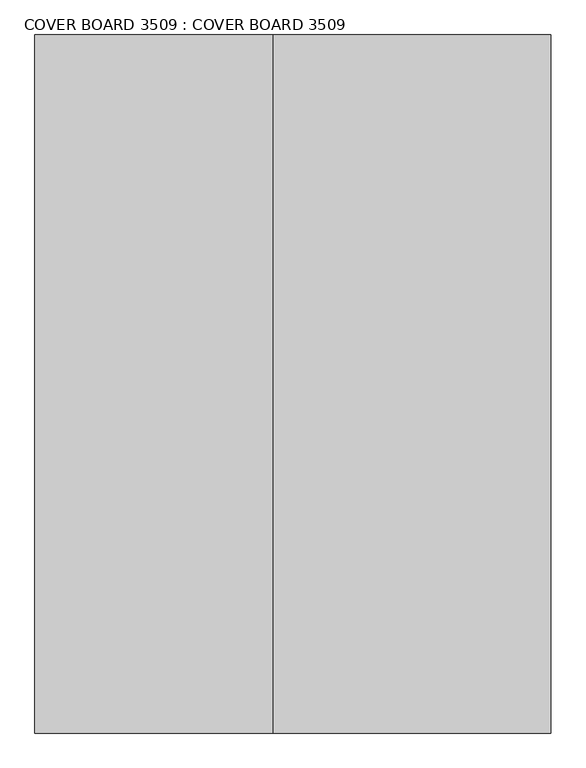
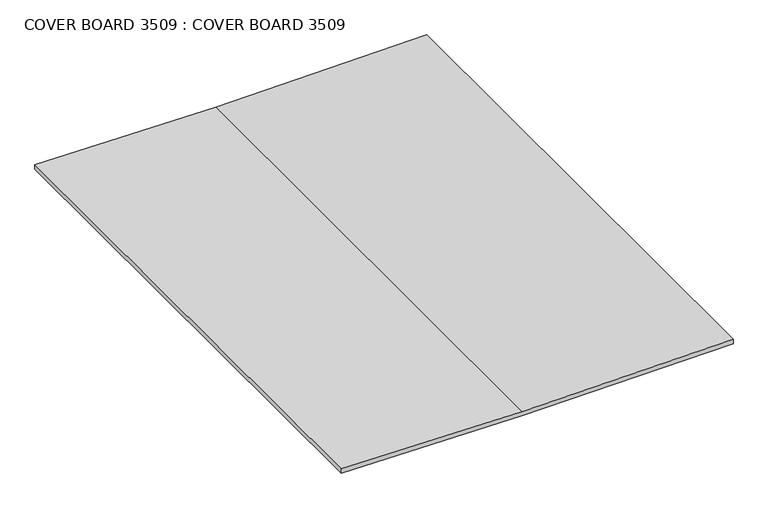
"""IFC4 building model written with IfcOpenShell, lengths in millimetres: proxy geometry, COVER BOARD 3509 : COVER BOARD 3509."""

from ifc_helpers import new_model, si_unit, frame, origin, place, context, project, spatial, polyline, outline, extrude, source, transform, mapped, element, save


def cover_board_3509_cover_board_3509_a2131a35(model_context):
    return source(origin(), model_context, "Body", "SweptSolid", [
        extrude(outline(polyline([(40228.1021556, -1886.5629484), (40237.9000089, -2567.3737014), (40220.5682898, -2567.3737014), (40210.7704365, -1886.5629484), (40220.5682898, -1090.0815411), (40237.9000089, -1090.0815411), (40228.1021556, -1886.5629484)])), frame((0.0, -1052.6406573, 0.0), z_axis=(0.0, 1.0, 0.0), x_axis=(0.0, 0.0, 1.0)), (0.0, 0.0, 1.0), 2000.0),
    ])


if __name__ == "__main__":
    model = new_model("IFC4")
    model_context = context("Model", 3, world=origin())
    ifc_project = project(units=[si_unit("LENGTHUNIT", "METRE", prefix="MILLI")], contexts=[model_context])
    site = spatial("IfcSite", under=ifc_project)
    building = spatial("IfcBuilding", under=site)
    placement = place(None, origin())
    cover_board_3509_cover_board_3509_shape = cover_board_3509_cover_board_3509_a2131a35(model_context)
    element("IfcBuildingElementProxy", 1, Name="COVER BOARD 3509 : COVER BOARD 3509", ObjectType="COVER BOARD 3509 : COVER BOARD 3509", at=placement, inside=building, context=model_context, shape_type="MappedRepresentation", body=[
        mapped(cover_board_3509_cover_board_3509_shape, transform((0.0, 0.0, 0.0), x_axis=(1.0, 0.0, 0.0), y_axis=(0.0, 1.0, 0.0), z_axis=(0.0, 0.0, 1.0))),
    ])
    save(model, "model.ifc")

# Revit data of these elements
# Type "COVER BOARD 3509 : COVER BOARD 3509"
#   NameOverride = "COVER BOARD"
# Element 1 (IfcBuildingElementProxy, "COVER BOARD 3509 : COVER BOARD 3509")
#   Materials on its faces: "CDX PLYWOOD - SEE STRUCTURAL DWGS"
# Materials
#   "CDX PLYWOOD - SEE STRUCTURAL DWGS": class "Unassigned", colour RGB 138 93 50, transparency 0, Cost = 0
